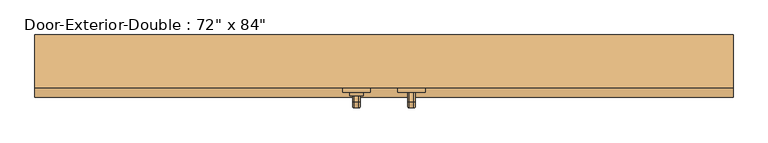
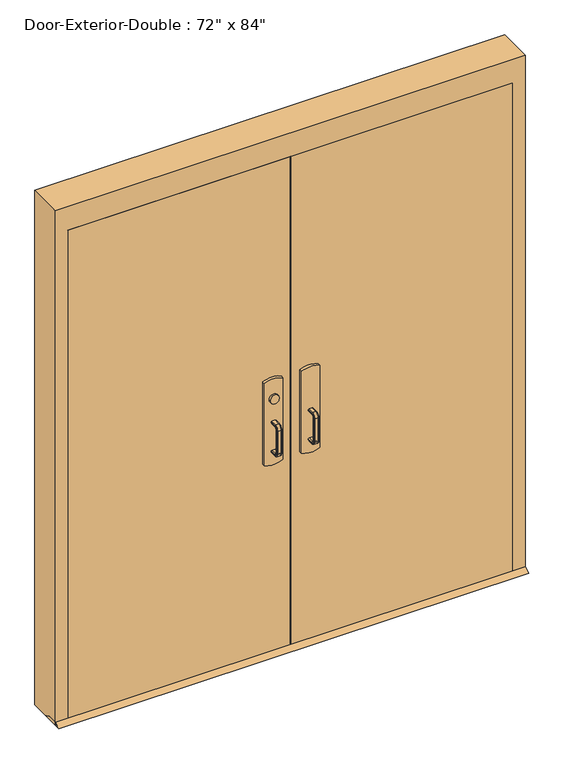
"""IFC4 building model written with IfcOpenShell, lengths in millimetres: door geometry."""

from ifc_helpers import new_model, si_unit, point, frame, frame_2d, origin, place, context, project, spatial, polyline, circle_curve, ellipse_curve, trimmed, segment, composite_curve, outline, extrude, faceted_brep, source, transform, mapped, element, save
from ifc_brep_helpers import plane_surface, cylinder_surface, revolved_surface, advanced_brep


def door_b0164ecf(model_context):
    return source(origin(), model_context, "Body", "SolidModel", [
        extrude(outline(polyline([(-575.7333333, 25.4), (-76.2, 25.4), (-76.2, 19.05), (-575.7333333, 19.05), (-575.7333333, 25.4)])), frame((0.0, 0.0, 990.6), z_axis=(0.0, 0.0, 1.0), x_axis=(1.0, 0.0, 0.0)), (0.0, 0.0, 1.0), 50.8),
        advanced_brep(
        [(-12.7, 19.05, 1041.4), (-12.7, 19.05, 990.6), (-76.2, 19.05, 990.6), (-825.5, 19.05, 990.6), (-825.5, 19.05, 1041.4), (-76.2, 19.05, 1041.4), (-825.5, -12.7, 1041.4), (-825.5, -12.7, 990.6), (-76.2, -12.7, 990.6), (-76.2, -12.7, 927.1), (-57.15, -12.7, 908.05), (-31.75, -12.7, 908.05), (-12.7, -12.7, 927.1), (-12.7, -12.7, 1104.9), (-31.75, -12.7, 1123.95), (-57.15, -12.7, 1123.95), (-76.2, -12.7, 1104.9), (-76.2, -12.7, 1041.4), (-76.2, 15.8747533, 1041.4), (-12.7, 15.8747533, 1041.4), (-12.7, 10.8645731, 1104.9), (-12.7, 10.8645731, 927.1), (-12.7, 15.8747533, 990.6), (-76.2, 15.8747533, 990.6), (-76.2, 10.8645731, 1104.9), (-76.2, 10.8645731, 927.1), (-31.75, 9.361519, 1123.95), (-57.15, 9.361519, 1123.95), (-57.15, 9.361519, 908.05), (-31.75, 9.361519, 908.05)],
        [
            (0, 1),
            (1, 2),
            (2, 3),
            (3, 4),
            (4, 5),
            (5, 0),
            (6, 7),
            (7, 8),
            (8, 9),
            (9, 10, circle_curve(frame((-57.15, -12.7, 927.1), z_axis=(0.0, -1.0, 0.0), x_axis=(-1.0, 0.0, 0.0)), 19.05)),
            (10, 11),
            (11, 12, circle_curve(frame((-31.75, -12.7, 927.1), z_axis=(0.0, -1.0, 0.0), x_axis=(-1.0, 0.0, 0.0)), 19.05)),
            (12, 13),
            (13, 14, circle_curve(frame((-31.75, -12.7, 1104.9), z_axis=(0.0, -1.0, 0.0), x_axis=(-1.0, 0.0, 0.0)), 19.05)),
            (14, 15),
            (15, 16, circle_curve(frame((-57.15, -12.7, 1104.9), z_axis=(0.0, -1.0, 0.0), x_axis=(-1.0, 0.0, 0.0)), 19.05)),
            (16, 17),
            (17, 6),
            (4, 6),
            (17, 18),
            (18, 19),
            (19, 0),
            (19, 20),
            (20, 13),
            (12, 21),
            (21, 22),
            (22, 1),
            (7, 3),
            (22, 23),
            (23, 8),
            (16, 24),
            (24, 18),
            (23, 25),
            (25, 9),
            (14, 26),
            (26, 27),
            (27, 15),
            (10, 28),
            (28, 29),
            (29, 11),
            (25, 28, ellipse_curve(frame((-57.15, 10.8645731, 927.1), z_axis=(0.0, -0.9969018152893365, 0.07865602756830282), x_axis=(0.0, 0.07865602756830208, 0.9969018152893365)), 19.1092038, 19.05)),
            (27, 24, ellipse_curve(frame((-57.15, 10.8645731, 1104.9), z_axis=(0.0, -0.9969018152893376, -0.07865602756828934), x_axis=(0.0, 0.078656027568288, -0.9969018152893377)), 19.1092038, 19.05)),
            (20, 26, ellipse_curve(frame((-31.75, 10.8645731, 1104.9), z_axis=(0.0, -0.9969018152893376, -0.07865602756828934), x_axis=(0.0, 0.078656027568288, -0.9969018152893377)), 19.1092038, 19.05)),
            (29, 21, ellipse_curve(frame((-31.75, 10.8645731, 927.1), z_axis=(0.0, -0.9969018152893365, 0.07865602756830282), x_axis=(0.0, 0.07865602756830208, 0.9969018152893365)), 19.1092038, 19.05)),
        ],
        [
            plane_surface(frame((-12.7, 19.05, 1041.4), z_axis=(0.0, 1.0, 0.0), x_axis=(1.0, 0.0, 0.0))),
            plane_surface(frame((-12.7, -12.7, 1041.4), z_axis=(0.0, -1.0, 0.0), x_axis=(-1.0, 0.0, 0.0))),
            plane_surface(frame((-825.5, 19.05, 1041.4), z_axis=(0.0, 0.0, 1.0), x_axis=(0.0, -1.0, 0.0))),
            plane_surface(frame((-12.7, 19.05, 1041.4), z_axis=(1.0, 0.0, 0.0), x_axis=(0.0, -1.0, 0.0))),
            plane_surface(frame((-12.7, 19.05, 990.6), z_axis=(0.0, 0.0, -1.0), x_axis=(0.0, -1.0, 0.0))),
            plane_surface(frame((-825.5, 19.05, 990.6), z_axis=(-1.0, 0.0, 0.0), x_axis=(0.0, -1.0, 0.0))),
            plane_surface(frame((-76.2, 15.8747533, 927.1), z_axis=(-1.0, 0.0, 0.0), x_axis=(0.0, -1.0, 0.0))),
            plane_surface(frame((-57.15, 15.8747533, 1123.95), z_axis=(0.0, 0.0, 1.0), x_axis=(0.0, -1.0, 0.0))),
            plane_surface(frame((-31.75, 15.8747533, 908.05), z_axis=(0.0, 0.0, -1.0), x_axis=(0.0, -1.0, 0.0))),
            cylinder_surface(frame((-57.15, -12.7, 927.1), z_axis=(0.0, 1.0, 0.0), x_axis=(-1.0, 0.0, 0.0)), 19.05),
            cylinder_surface(frame((-57.15, -12.7, 1104.9), z_axis=(0.0, 1.0, 0.0), x_axis=(-1.0, 0.0, 0.0)), 19.05),
            cylinder_surface(frame((-31.75, -12.7, 1104.9), z_axis=(0.0, 1.0, 0.0), x_axis=(-1.0, 0.0, 0.0)), 19.05),
            cylinder_surface(frame((-31.75, -12.7, 927.1), z_axis=(0.0, 1.0, 0.0), x_axis=(-1.0, 0.0, 0.0)), 19.05),
            plane_surface(frame((-76.2, 15.8747533, 1041.4), z_axis=(0.0, 0.9969018152893376, 0.07865602756828934), x_axis=(1.0, 0.0, 0.0))),
            plane_surface(frame((-76.2, 9.361519, 908.05), z_axis=(0.0, 0.9969018152893365, -0.07865602756830282), x_axis=(1.0, 0.0, 0.0))),
        ],
        [
            (0, [[1, 2, 3, 4, 5, 6]]),
            (1, [[7, 8, 9, 10, 11, 12, 13, 14, 15, 16, 17, 18]]),
            (2, [[19, -18, 20, 21, 22, -6, -5]]),
            (3, [[-1, -22, 23, 24, -13, 25, 26, 27]]),
            (4, [[28, -3, -2, -27, 29, 30, -8]]),
            (5, [[-4, -28, -7, -19]]),
            (6, [[-17, 31, 32, -20]]),
            (6, [[-9, -30, 33, 34]]),
            (7, [[-15, 35, 36, 37]]),
            (8, [[-11, 38, 39, 40]]),
            (9, [[-10, -34, 41, -38]]),
            (10, [[-16, -37, 42, -31]]),
            (11, [[-14, -24, 43, -35]]),
            (12, [[-12, -40, 44, -25]]),
            (13, [[-21, -32, -42, -36, -43, -23]]),
            (14, [[-26, -44, -39, -41, -33, -29]]),
        ],
    ),
        extrude(outline(polyline([(-57.15, 12.7), (-12.7, 12.7), (12.7, 0.0), (-82.55, 0.0), (-57.15, 12.7)])), frame((-965.2, 0.0, 0.0), z_axis=(1.0, 0.0, 0.0), x_axis=(0.0, 1.0, 0.0)), (0.0, 0.0, 1.0), 1930.4),
        extrude(outline(polyline([(575.7333333, 25.4), (575.7333333, 19.05), (76.2, 19.05), (76.2, 25.4), (575.7333333, 25.4)])), frame((0.0, 0.0, 990.6), z_axis=(0.0, 0.0, 1.0), x_axis=(1.0, 0.0, 0.0)), (0.0, 0.0, 1.0), 50.8),
        advanced_brep(
        [(12.7, 19.05, 1041.4), (76.2, 19.05, 1041.4), (825.5, 19.05, 1041.4), (825.5, 19.05, 990.6), (76.2, 19.05, 990.6), (12.7, 19.05, 990.6), (825.5, -12.7, 1041.4), (76.2, -12.7, 1041.4), (76.2, -12.7, 1104.9), (57.15, -12.7, 1123.95), (31.75, -12.7, 1123.95), (12.7, -12.7, 1104.9), (12.7, -12.7, 927.1), (31.75, -12.7, 908.05), (57.15, -12.7, 908.05), (76.2, -12.7, 927.1), (76.2, -12.7, 990.6), (825.5, -12.7, 990.6), (12.7, 15.8747533, 1041.4), (76.2, 15.8747533, 1041.4), (12.7, 15.8747533, 990.6), (12.7, 10.8645731, 927.1), (12.7, 10.8645731, 1104.9), (76.2, 15.8747533, 990.6), (76.2, 10.8645731, 1104.9), (76.2, 10.8645731, 927.1), (57.15, 9.361519, 1123.95), (31.75, 9.361519, 1123.95), (31.75, 9.361519, 908.05), (57.15, 9.361519, 908.05)],
        [
            (0, 1),
            (1, 2),
            (2, 3),
            (3, 4),
            (4, 5),
            (5, 0),
            (6, 7),
            (7, 8),
            (8, 9, circle_curve(frame((57.15, -12.7, 1104.9), z_axis=(0.0, -1.0, 0.0), x_axis=(1.0, 0.0, 0.0)), 19.05)),
            (9, 10),
            (10, 11, circle_curve(frame((31.75, -12.7, 1104.9), z_axis=(0.0, -1.0, 0.0), x_axis=(1.0, 0.0, 0.0)), 19.05)),
            (11, 12),
            (12, 13, circle_curve(frame((31.75, -12.7, 927.1), z_axis=(0.0, -1.0, 0.0), x_axis=(1.0, 0.0, 0.0)), 19.05)),
            (13, 14),
            (14, 15, circle_curve(frame((57.15, -12.7, 927.1), z_axis=(0.0, -1.0, 0.0), x_axis=(1.0, 0.0, 0.0)), 19.05)),
            (15, 16),
            (16, 17),
            (17, 6),
            (0, 18),
            (18, 19),
            (19, 7),
            (6, 2),
            (5, 20),
            (20, 21),
            (21, 12),
            (11, 22),
            (22, 18),
            (16, 23),
            (23, 20),
            (3, 17),
            (19, 24),
            (24, 8),
            (15, 25),
            (25, 23),
            (9, 26),
            (26, 27),
            (27, 10),
            (13, 28),
            (28, 29),
            (29, 14),
            (29, 25, ellipse_curve(frame((57.15, 10.8645731, 927.1), z_axis=(0.0, -0.9969018152893365, 0.07865602756830282), x_axis=(0.0, 0.07865602756830208, 0.9969018152893365)), 19.1092038, 19.05)),
            (24, 26, ellipse_curve(frame((57.15, 10.8645731, 1104.9), z_axis=(0.0, -0.9969018152893376, -0.07865602756828934), x_axis=(0.0, 0.078656027568288, -0.9969018152893377)), 19.1092038, 19.05)),
            (27, 22, ellipse_curve(frame((31.75, 10.8645731, 1104.9), z_axis=(0.0, -0.9969018152893376, -0.07865602756828934), x_axis=(0.0, 0.078656027568288, -0.9969018152893377)), 19.1092038, 19.05)),
            (21, 28, ellipse_curve(frame((31.75, 10.8645731, 927.1), z_axis=(0.0, -0.9969018152893365, 0.07865602756830282), x_axis=(0.0, 0.07865602756830208, 0.9969018152893365)), 19.1092038, 19.05)),
        ],
        [
            plane_surface(frame((12.7, 19.05, 1041.4), z_axis=(0.0, 1.0, 0.0), x_axis=(-1.0, 0.0, 0.0))),
            plane_surface(frame((12.7, -12.7, 1041.4), z_axis=(0.0, -1.0, 0.0), x_axis=(1.0, 0.0, 0.0))),
            plane_surface(frame((825.5, 19.05, 1041.4), z_axis=(0.0, 0.0, 1.0), x_axis=(0.0, -1.0, 0.0))),
            plane_surface(frame((12.7, 19.05, 1041.4), z_axis=(-1.0, 0.0, 0.0), x_axis=(0.0, -1.0, 0.0))),
            plane_surface(frame((12.7, 19.05, 990.6), z_axis=(0.0, 0.0, -1.0), x_axis=(0.0, -1.0, 0.0))),
            plane_surface(frame((825.5, 19.05, 990.6), z_axis=(1.0, 0.0, 0.0), x_axis=(0.0, -1.0, 0.0))),
            plane_surface(frame((76.2, 15.8747533, 927.1), z_axis=(1.0, 0.0, 0.0), x_axis=(0.0, -1.0, 0.0))),
            plane_surface(frame((57.15, 15.8747533, 1123.95), z_axis=(0.0, 0.0, 1.0), x_axis=(0.0, -1.0, 0.0))),
            plane_surface(frame((31.75, 15.8747533, 908.05), z_axis=(0.0, 0.0, -1.0), x_axis=(0.0, -1.0, 0.0))),
            cylinder_surface(frame((57.15, -12.7, 927.1), z_axis=(0.0, 1.0, 0.0), x_axis=(1.0, 0.0, 0.0)), 19.05),
            cylinder_surface(frame((57.15, -12.7, 1104.9), z_axis=(0.0, 1.0, 0.0), x_axis=(1.0, 0.0, 0.0)), 19.05),
            cylinder_surface(frame((31.75, -12.7, 1104.9), z_axis=(0.0, 1.0, 0.0), x_axis=(1.0, 0.0, 0.0)), 19.05),
            cylinder_surface(frame((31.75, -12.7, 927.1), z_axis=(0.0, 1.0, 0.0), x_axis=(1.0, 0.0, 0.0)), 19.05),
            plane_surface(frame((76.2, 15.8747533, 1041.4), z_axis=(0.0, 0.9969018152893376, 0.07865602756828934), x_axis=(-1.0, 0.0, 0.0))),
            plane_surface(frame((76.2, 9.361519, 908.05), z_axis=(0.0, 0.9969018152893365, -0.07865602756830282), x_axis=(-1.0, 0.0, 0.0))),
        ],
        [
            (0, [[1, 2, 3, 4, 5, 6]]),
            (1, [[7, 8, 9, 10, 11, 12, 13, 14, 15, 16, 17, 18]]),
            (2, [[-2, -1, 19, 20, 21, -7, 22]]),
            (3, [[23, 24, 25, -12, 26, 27, -19, -6]]),
            (4, [[-17, 28, 29, -23, -5, -4, 30]]),
            (5, [[-22, -18, -30, -3]]),
            (6, [[-21, 31, 32, -8]]),
            (6, [[33, 34, -28, -16]]),
            (7, [[35, 36, 37, -10]]),
            (8, [[38, 39, 40, -14]]),
            (9, [[-40, 41, -33, -15]]),
            (10, [[-32, 42, -35, -9]]),
            (11, [[-37, 43, -26, -11]]),
            (12, [[-25, 44, -38, -13]]),
            (13, [[-27, -43, -36, -42, -31, -20]]),
            (14, [[-29, -34, -41, -39, -44, -24]]),
        ],
    ),
        advanced_brep(
        [(66.2, -69.85, 1017.190625), (69.771875, -69.85, 1020.7625), (82.628125, -69.85, 1020.7625), (86.2, -69.85, 1017.190625), (86.2, -69.85, 1014.8090406), (82.6284594, -69.85, 1011.2375), (69.771875, -69.85, 1011.2375), (66.2, -69.85, 1014.809375), (66.2, -69.85, 887.809375), (66.2, -69.85, 890.190625), (69.771875, -69.85, 893.7625), (82.6284594, -69.85, 893.7625), (86.2, -69.85, 890.1909594), (86.2, -69.85, 887.809375), (82.628125, -69.85, 884.2375), (69.771875, -69.85, 884.2375), (66.2, -95.25, 1014.809375), (66.2, -106.759375, 1003.3), (66.2, -106.759375, 901.7), (66.2, -95.25, 890.190625), (66.2, -95.25, 887.809375), (66.2, -109.140625, 901.7), (66.2, -109.140625, 1003.3), (66.2, -95.25, 1017.190625), (69.771875, -95.25, 1011.2375), (82.6284594, -95.25, 1011.2375), (86.2, -95.25, 1014.8090406), (86.2, -95.25, 1017.190625), (86.2, -109.140625, 1003.3), (86.2, -109.140625, 901.7), (86.2, -95.25, 887.809375), (86.2, -95.25, 890.1909594), (86.2, -106.7590406, 901.7), (86.2, -106.7590406, 1003.3), (82.628125, -95.25, 1020.7625), (69.771875, -95.25, 1020.7625), (69.771875, -103.1875, 1003.3), (82.6284594, -103.1875, 1003.3), (82.628125, -112.7125, 1003.3), (69.771875, -112.7125, 1003.3), (69.771875, -103.1875, 901.7), (82.6284594, -103.1875, 901.7), (82.628125, -112.7125, 901.7), (69.771875, -112.7125, 901.7), (69.771875, -95.25, 893.7625), (82.6284594, -95.25, 893.7625), (82.628125, -95.25, 884.2375), (69.771875, -95.25, 884.2375)],
        [
            (0, 1, circle_curve(frame((69.771875, -69.85, 1017.190625), z_axis=(0.0, 1.0, 0.0), x_axis=(0.0, 0.0, 1.0)), 3.571875)),
            (1, 2),
            (2, 3, circle_curve(frame((82.628125, -69.85, 1017.190625), z_axis=(0.0, 1.0, 0.0), x_axis=(0.0, 0.0, 1.0)), 3.571875)),
            (3, 4),
            (4, 5, circle_curve(frame((82.6284594, -69.85, 1014.8090406), z_axis=(0.0, 1.0, 0.0), x_axis=(0.0, 0.0, 1.0)), 3.5715406)),
            (5, 6),
            (6, 7, circle_curve(frame((69.771875, -69.85, 1014.809375), z_axis=(0.0, 1.0, 0.0), x_axis=(0.0, 0.0, 1.0)), 3.571875)),
            (7, 0),
            (8, 9),
            (9, 10, circle_curve(frame((69.771875, -69.85, 890.190625), z_axis=(0.0, 1.0, 0.0), x_axis=(0.0, 0.0, -1.0)), 3.571875)),
            (10, 11),
            (11, 12, circle_curve(frame((82.6284594, -69.85, 890.1909594), z_axis=(0.0, 1.0, 0.0), x_axis=(0.0, 0.0, -1.0)), 3.5715406)),
            (12, 13),
            (13, 14, circle_curve(frame((82.628125, -69.85, 887.809375), z_axis=(0.0, 1.0, 0.0), x_axis=(0.0, 0.0, -1.0)), 3.571875)),
            (14, 15),
            (15, 8, circle_curve(frame((69.771875, -69.85, 887.809375), z_axis=(0.0, 1.0, 0.0), x_axis=(0.0, 0.0, -1.0)), 3.571875)),
            (7, 16),
            (16, 17, circle_curve(frame((66.2, -95.25, 1003.3), z_axis=(1.0, 0.0, 0.0), x_axis=(0.0, 0.0, 1.0)), 11.509375)),
            (17, 18),
            (18, 19, circle_curve(frame((66.2, -95.25, 901.7), z_axis=(1.0, 0.0, 0.0), x_axis=(0.0, -1.0, 0.0)), 11.509375)),
            (19, 9),
            (8, 20),
            (20, 21, circle_curve(frame((66.2, -95.25, 901.7), z_axis=(-1.0, 0.0, 0.0), x_axis=(0.0, -1.0, 0.0)), 13.890625)),
            (21, 22),
            (22, 23, circle_curve(frame((66.2, -95.25, 1003.3), z_axis=(-1.0, 0.0, 0.0), x_axis=(0.0, 0.0, 1.0)), 13.890625)),
            (23, 0),
            (6, 24),
            (24, 16, circle_curve(frame((69.771875, -95.25, 1014.809375), z_axis=(0.0, 1.0, 0.0), x_axis=(0.0, 0.0, 1.0)), 3.571875)),
            (5, 25),
            (25, 24),
            (4, 26),
            (26, 25, circle_curve(frame((82.6284594, -95.25, 1014.8090406), z_axis=(0.0, 1.0, 0.0), x_axis=(0.0, 0.0, 1.0)), 3.5715406)),
            (3, 27),
            (27, 28, circle_curve(frame((86.2, -95.25, 1003.3), z_axis=(1.0, 0.0, 0.0), x_axis=(0.0, 0.0, 1.0)), 13.890625)),
            (28, 29),
            (29, 30, circle_curve(frame((86.2, -95.25, 901.7), z_axis=(1.0, 0.0, 0.0), x_axis=(0.0, -1.0, 0.0)), 13.890625)),
            (30, 13),
            (12, 31),
            (31, 32, circle_curve(frame((86.2, -95.25, 901.7), z_axis=(-1.0, 0.0, 0.0), x_axis=(0.0, -1.0, 0.0)), 11.5090406)),
            (32, 33),
            (33, 26, circle_curve(frame((86.2, -95.25, 1003.3), z_axis=(-1.0, 0.0, 0.0), x_axis=(0.0, 0.0, 1.0)), 11.5090406)),
            (2, 34),
            (34, 27, circle_curve(frame((82.628125, -95.25, 1017.190625), z_axis=(0.0, 1.0, 0.0), x_axis=(0.0, 0.0, 1.0)), 3.571875)),
            (1, 35),
            (35, 34),
            (23, 35, circle_curve(frame((69.771875, -95.25, 1017.190625), z_axis=(0.0, 1.0, 0.0), x_axis=(0.0, 0.0, 1.0)), 3.571875)),
            (36, 17, circle_curve(frame((69.771875, -106.759375, 1003.3), z_axis=(0.0, 0.0, 1.0), x_axis=(0.0, -1.0, 0.0)), 3.571875)),
            (24, 36, circle_curve(frame((69.771875, -95.25, 1003.3), z_axis=(1.0, 0.0, 0.0), x_axis=(0.0, 0.0, 1.0)), 7.9375)),
            (37, 36),
            (25, 37, circle_curve(frame((82.6284594, -95.25, 1003.3), z_axis=(1.0, 0.0, 0.0), x_axis=(0.0, 0.0, 1.0)), 7.9375)),
            (33, 37, circle_curve(frame((82.6284594, -106.7590406, 1003.3), z_axis=(0.0, 0.0, 1.0), x_axis=(0.0, -1.0, 0.0)), 3.5715406)),
            (38, 28, circle_curve(frame((82.628125, -109.140625, 1003.3), z_axis=(0.0, 0.0, 1.0), x_axis=(0.0, -1.0, 0.0)), 3.571875)),
            (34, 38, circle_curve(frame((82.628125, -95.25, 1003.3), z_axis=(1.0, 0.0, 0.0), x_axis=(0.0, 0.0, 1.0)), 17.4625)),
            (39, 38),
            (35, 39, circle_curve(frame((69.771875, -95.25, 1003.3), z_axis=(1.0, 0.0, 0.0), x_axis=(0.0, 0.0, 1.0)), 17.4625)),
            (22, 39, circle_curve(frame((69.771875, -109.140625, 1003.3), z_axis=(0.0, 0.0, 1.0), x_axis=(0.0, -1.0, 0.0)), 3.571875)),
            (36, 40),
            (40, 18, circle_curve(frame((69.771875, -106.759375, 901.7), z_axis=(0.0, 0.0, 1.0), x_axis=(0.0, -1.0, 0.0)), 3.571875)),
            (37, 41),
            (41, 40),
            (32, 41, circle_curve(frame((82.6284594, -106.7590406, 901.7), z_axis=(0.0, 0.0, 1.0), x_axis=(0.0, -1.0, 0.0)), 3.5715406)),
            (38, 42),
            (42, 29, circle_curve(frame((82.628125, -109.140625, 901.7), z_axis=(0.0, 0.0, 1.0), x_axis=(0.0, -1.0, 0.0)), 3.571875)),
            (39, 43),
            (43, 42),
            (21, 43, circle_curve(frame((69.771875, -109.140625, 901.7), z_axis=(0.0, 0.0, 1.0), x_axis=(0.0, -1.0, 0.0)), 3.571875)),
            (44, 19, circle_curve(frame((69.771875, -95.25, 890.190625), z_axis=(0.0, -1.0, 0.0), x_axis=(0.0, 0.0, -1.0)), 3.571875)),
            (40, 44, circle_curve(frame((69.771875, -95.25, 901.7), z_axis=(1.0, 0.0, 0.0), x_axis=(0.0, -1.0, 0.0)), 7.9375)),
            (45, 44),
            (41, 45, circle_curve(frame((82.6284594, -95.25, 901.7), z_axis=(1.0, 0.0, 0.0), x_axis=(0.0, -1.0, 0.0)), 7.9375)),
            (31, 45, circle_curve(frame((82.6284594, -95.25, 890.1909594), z_axis=(0.0, -1.0, 0.0), x_axis=(0.0, 0.0, -1.0)), 3.5715406)),
            (46, 30, circle_curve(frame((82.628125, -95.25, 887.809375), z_axis=(0.0, -1.0, 0.0), x_axis=(0.0, 0.0, -1.0)), 3.571875)),
            (42, 46, circle_curve(frame((82.628125, -95.25, 901.7), z_axis=(1.0, 0.0, 0.0), x_axis=(0.0, -1.0, 0.0)), 17.4625)),
            (47, 46),
            (43, 47, circle_curve(frame((69.771875, -95.25, 901.7), z_axis=(1.0, 0.0, 0.0), x_axis=(0.0, -1.0, 0.0)), 17.4625)),
            (20, 47, circle_curve(frame((69.771875, -95.25, 887.809375), z_axis=(0.0, -1.0, 0.0), x_axis=(0.0, 0.0, -1.0)), 3.571875)),
            (44, 10),
            (45, 11),
            (46, 14),
            (47, 15),
        ],
        [
            plane_surface(frame((76.2, -69.85, 1016.0), z_axis=(0.0, 1.0, 0.0), x_axis=(1.0, 0.0, 0.0))),
            plane_surface(frame((76.2, -69.85, 889.0), z_axis=(0.0, 1.0, 0.0), x_axis=(1.0, 0.0, 0.0))),
            plane_surface(frame((66.2, -69.85, 1017.190625), z_axis=(-1.0, 0.0, 0.0), x_axis=(0.0, -1.0, 0.0))),
            cylinder_surface(frame((69.771875, -69.85, 1014.809375), z_axis=(0.0, 1.0, 0.0), x_axis=(0.0, 0.0, 1.0)), 3.571875),
            plane_surface(frame((69.771875, -69.85, 1011.2375), z_axis=(0.0, 0.0, -1.0), x_axis=(0.0, -1.0, 0.0))),
            cylinder_surface(frame((82.6284594, -69.85, 1014.8090406), z_axis=(0.0, 1.0, 0.0), x_axis=(0.0, 0.0, 1.0)), 3.5715406),
            plane_surface(frame((86.2, -69.85, 1014.8090406), z_axis=(1.0, 0.0, 0.0), x_axis=(0.0, -1.0, 0.0))),
            cylinder_surface(frame((82.628125, -69.85, 1017.190625), z_axis=(0.0, 1.0, 0.0), x_axis=(0.0, 0.0, 1.0)), 3.571875),
            plane_surface(frame((82.628125, -69.85, 1020.7625), z_axis=(0.0, 0.0, 1.0), x_axis=(0.0, -1.0, 0.0))),
            cylinder_surface(frame((69.771875, -69.85, 1017.190625), z_axis=(0.0, 1.0, 0.0), x_axis=(0.0, 0.0, 1.0)), 3.571875),
            revolved_surface(trimmed(ellipse_curve(frame((69.771875, -95.25, 1014.809375), z_axis=(0.0, -1.0, 0.0), x_axis=(0.0, 0.0, 1.0)), 3.571875, 3.571875), [point((66.2, -95.25, 1014.809375))], [point((69.771875, -95.25, 1011.2375))], True, "CARTESIAN"), (76.2, -95.25, 1003.3), (-1.0, 0.0, 0.0)),
            revolved_surface(polyline([(69.771875, -95.25, 1011.2375), (82.6284594, -95.25, 1011.2375)]), (76.2, -95.25, 1003.3), (-1.0, 0.0, 0.0)),
            revolved_surface(trimmed(ellipse_curve(frame((82.6284594, -95.25, 1014.8090406), z_axis=(0.0, -1.0, 0.0), x_axis=(0.0, 0.0, 1.0)), 3.5715406, 3.5715406), [point((82.6284594, -95.25, 1011.2375))], [point((86.2, -95.25, 1014.8090406))], True, "CARTESIAN"), (76.2, -95.25, 1003.3), (-1.0, 0.0, 0.0)),
            revolved_surface(trimmed(ellipse_curve(frame((82.628125, -95.25, 1017.190625), z_axis=(0.0, -1.0, 0.0), x_axis=(0.0, 0.0, 1.0)), 3.571875, 3.571875), [point((86.2, -95.25, 1017.190625))], [point((82.628125, -95.25, 1020.7625))], True, "CARTESIAN"), (76.2, -95.25, 1003.3), (-1.0, 0.0, 0.0)),
            cylinder_surface(frame((76.2, -95.25, 1003.3), z_axis=(-1.0, 0.0, 0.0), x_axis=(0.0, 0.0, 1.0)), 17.4625),
            revolved_surface(trimmed(ellipse_curve(frame((69.771875, -95.25, 1017.190625), z_axis=(0.0, -1.0, 0.0), x_axis=(0.0, 0.0, 1.0)), 3.571875, 3.571875), [point((69.771875, -95.25, 1020.7625))], [point((66.2, -95.25, 1017.190625))], True, "CARTESIAN"), (76.2, -95.25, 1003.3), (-1.0, 0.0, 0.0)),
            cylinder_surface(frame((69.771875, -106.759375, 1003.3), z_axis=(0.0, 0.0, 1.0), x_axis=(0.0, -1.0, 0.0)), 3.571875),
            plane_surface(frame((69.771875, -103.1875, 1003.3), z_axis=(0.0, 1.0, 0.0), x_axis=(0.0, 0.0, -1.0))),
            cylinder_surface(frame((82.6284594, -106.7590406, 1003.3), z_axis=(0.0, 0.0, 1.0), x_axis=(0.0, -1.0, 0.0)), 3.5715406),
            cylinder_surface(frame((82.628125, -109.140625, 1003.3), z_axis=(0.0, 0.0, 1.0), x_axis=(0.0, -1.0, 0.0)), 3.571875),
            plane_surface(frame((82.628125, -112.7125, 1003.3), z_axis=(0.0, -1.0, 0.0), x_axis=(0.0, 0.0, -1.0))),
            cylinder_surface(frame((69.771875, -109.140625, 1003.3), z_axis=(0.0, 0.0, 1.0), x_axis=(0.0, -1.0, 0.0)), 3.571875),
            revolved_surface(trimmed(ellipse_curve(frame((69.771875, -106.759375, 901.7), z_axis=(0.0, 0.0, -1.0), x_axis=(0.0, -1.0, 0.0)), 3.571875, 3.571875), [point((66.2, -106.759375, 901.7))], [point((69.771875, -103.1875, 901.7))], True, "CARTESIAN"), (76.2, -95.25, 901.7), (-1.0, 0.0, 0.0)),
            revolved_surface(polyline([(69.771875, -103.1875, 901.7), (82.6284594, -103.1875, 901.7)]), (76.2, -95.25, 901.7), (-1.0, 0.0, 0.0)),
            revolved_surface(trimmed(ellipse_curve(frame((82.6284594, -106.7590406, 901.7), z_axis=(0.0, 0.0, -1.0), x_axis=(0.0, -1.0, 0.0)), 3.5715406, 3.5715406), [point((82.6284594, -103.1875, 901.7))], [point((86.2, -106.7590406, 901.7))], True, "CARTESIAN"), (76.2, -95.25, 901.7), (-1.0, 0.0, 0.0)),
            revolved_surface(trimmed(ellipse_curve(frame((82.628125, -109.140625, 901.7), z_axis=(0.0, 0.0, -1.0), x_axis=(0.0, -1.0, 0.0)), 3.571875, 3.571875), [point((86.2, -109.140625, 901.7))], [point((82.628125, -112.7125, 901.7))], True, "CARTESIAN"), (76.2, -95.25, 901.7), (-1.0, 0.0, 0.0)),
            cylinder_surface(frame((76.2, -95.25, 901.7), z_axis=(-1.0, 0.0, 0.0), x_axis=(0.0, -1.0, 0.0)), 17.4625),
            revolved_surface(trimmed(ellipse_curve(frame((69.771875, -109.140625, 901.7), z_axis=(0.0, 0.0, -1.0), x_axis=(0.0, -1.0, 0.0)), 3.571875, 3.571875), [point((69.771875, -112.7125, 901.7))], [point((66.2, -109.140625, 901.7))], True, "CARTESIAN"), (76.2, -95.25, 901.7), (-1.0, 0.0, 0.0)),
            cylinder_surface(frame((69.771875, -95.25, 890.190625), z_axis=(0.0, -1.0, 0.0), x_axis=(0.0, 0.0, -1.0)), 3.571875),
            plane_surface(frame((69.771875, -95.25, 893.7625), z_axis=(0.0, 0.0, 1.0), x_axis=(0.0, 1.0, 0.0))),
            cylinder_surface(frame((82.6284594, -95.25, 890.1909594), z_axis=(0.0, -1.0, 0.0), x_axis=(0.0, 0.0, -1.0)), 3.5715406),
            cylinder_surface(frame((82.628125, -95.25, 887.809375), z_axis=(0.0, -1.0, 0.0), x_axis=(0.0, 0.0, -1.0)), 3.571875),
            plane_surface(frame((82.628125, -95.25, 884.2375), z_axis=(0.0, 0.0, -1.0), x_axis=(0.0, 1.0, 0.0))),
            cylinder_surface(frame((69.771875, -95.25, 887.809375), z_axis=(0.0, -1.0, 0.0), x_axis=(0.0, 0.0, -1.0)), 3.571875),
        ],
        [
            (0, [[1, 2, 3, 4, 5, 6, 7, 8]]),
            (1, [[9, 10, 11, 12, 13, 14, 15, 16]]),
            (2, [[17, 18, 19, 20, 21, -9, 22, 23, 24, 25, 26, -8]]),
            (3, [[27, 28, -17, -7]]),
            (4, [[29, 30, -27, -6]]),
            (5, [[31, 32, -29, -5]]),
            (6, [[33, 34, 35, 36, 37, -13, 38, 39, 40, 41, -31, -4]]),
            (7, [[42, 43, -33, -3]]),
            (8, [[44, 45, -42, -2]]),
            (9, [[-26, 46, -44, -1]]),
            (10, [[47, -18, -28, 48]]),
            (11, [[49, -48, -30, 50]]),
            (12, [[51, -50, -32, -41]]),
            (13, [[52, -34, -43, 53]]),
            (14, [[54, -53, -45, 55]]),
            (15, [[56, -55, -46, -25]]),
            (16, [[57, 58, -19, -47]]),
            (17, [[59, 60, -57, -49]]),
            (18, [[-40, 61, -59, -51]]),
            (19, [[62, 63, -35, -52]]),
            (20, [[64, 65, -62, -54]]),
            (21, [[-24, 66, -64, -56]]),
            (22, [[67, -20, -58, 68]]),
            (23, [[69, -68, -60, 70]]),
            (24, [[71, -70, -61, -39]]),
            (25, [[72, -36, -63, 73]]),
            (26, [[74, -73, -65, 75]]),
            (27, [[76, -75, -66, -23]]),
            (28, [[77, -10, -21, -67]]),
            (29, [[78, -11, -77, -69]]),
            (30, [[-38, -12, -78, -71]]),
            (31, [[79, -14, -37, -72]]),
            (32, [[80, -15, -79, -74]]),
            (33, [[-22, -16, -80, -76]]),
        ],
    ),
        extrude(outline(composite_curve([segment(trimmed(circle_curve(frame_2d((1113.0338574, 76.2)), 89.3016225), [point((1193.8, 114.3))], [point((1193.8, 38.1))], False, "CARTESIAN"), True, "CONTINUOUS"), segment(polyline([(1193.8, 38.1), (838.2, 38.1)]), True, "CONTINUOUS"), segment(trimmed(circle_curve(frame_2d((918.9661426, 76.2)), 89.3016225), [point((838.2, 38.1))], [point((838.2, 114.3))], False, "CARTESIAN"), True, "CONTINUOUS"), segment(polyline([(838.2, 114.3), (1193.8, 114.3)]), True, "CONTINUOUS")], self_intersect=False)), frame((0.0, -69.85, 0.0), z_axis=(0.0, 1.0, 0.0), x_axis=(0.0, 0.0, 1.0)), (0.0, 0.0, 1.0), 12.7),
        advanced_brep(
        [(-86.2, -69.85, 1017.190625), (-82.628125, -69.85, 1020.7625), (-69.771875, -69.85, 1020.7625), (-66.2, -69.85, 1017.190625), (-66.2, -69.85, 1014.8090406), (-69.7715406, -69.85, 1011.2375), (-82.628125, -69.85, 1011.2375), (-86.2, -69.85, 1014.809375), (-86.2, -69.85, 887.809375), (-86.2, -69.85, 890.190625), (-82.628125, -69.85, 893.7625), (-69.7715406, -69.85, 893.7625), (-66.2, -69.85, 890.1909594), (-66.2, -69.85, 887.809375), (-69.771875, -69.85, 884.2375), (-82.628125, -69.85, 884.2375), (-86.2, -95.25, 1014.809375), (-86.2, -106.759375, 1003.3), (-86.2, -106.759375, 901.7), (-86.2, -95.25, 890.190625), (-86.2, -95.25, 887.809375), (-86.2, -109.140625, 901.7), (-86.2, -109.140625, 1003.3), (-86.2, -95.25, 1017.190625), (-82.628125, -95.25, 1011.2375), (-69.7715406, -95.25, 1011.2375), (-66.2, -95.25, 1014.8090406), (-66.2, -95.25, 1017.190625), (-66.2, -109.140625, 1003.3), (-66.2, -109.140625, 901.7), (-66.2, -95.25, 887.809375), (-66.2, -95.25, 890.1909594), (-66.2, -106.7590406, 901.7), (-66.2, -106.7590406, 1003.3), (-69.771875, -95.25, 1020.7625), (-82.628125, -95.25, 1020.7625), (-82.628125, -103.1875, 1003.3), (-69.7715406, -103.1875, 1003.3), (-69.771875, -112.7125, 1003.3), (-82.628125, -112.7125, 1003.3), (-82.628125, -103.1875, 901.7), (-69.7715406, -103.1875, 901.7), (-69.771875, -112.7125, 901.7), (-82.628125, -112.7125, 901.7), (-82.628125, -95.25, 893.7625), (-69.7715406, -95.25, 893.7625), (-69.771875, -95.25, 884.2375), (-82.628125, -95.25, 884.2375)],
        [
            (0, 1, circle_curve(frame((-82.628125, -69.85, 1017.190625), z_axis=(0.0, 1.0, 0.0), x_axis=(0.0, 0.0, 1.0)), 3.571875)),
            (1, 2),
            (2, 3, circle_curve(frame((-69.771875, -69.85, 1017.190625), z_axis=(0.0, 1.0, 0.0), x_axis=(0.0, 0.0, 1.0)), 3.571875)),
            (3, 4),
            (4, 5, circle_curve(frame((-69.7715406, -69.85, 1014.8090406), z_axis=(0.0, 1.0, 0.0), x_axis=(0.0, 0.0, 1.0)), 3.5715406)),
            (5, 6),
            (6, 7, circle_curve(frame((-82.628125, -69.85, 1014.809375), z_axis=(0.0, 1.0, 0.0), x_axis=(0.0, 0.0, 1.0)), 3.571875)),
            (7, 0),
            (8, 9),
            (9, 10, circle_curve(frame((-82.628125, -69.85, 890.190625), z_axis=(0.0, 1.0, 0.0), x_axis=(0.0, 0.0, -1.0)), 3.571875)),
            (10, 11),
            (11, 12, circle_curve(frame((-69.7715406, -69.85, 890.1909594), z_axis=(0.0, 1.0, 0.0), x_axis=(0.0, 0.0, -1.0)), 3.5715406)),
            (12, 13),
            (13, 14, circle_curve(frame((-69.771875, -69.85, 887.809375), z_axis=(0.0, 1.0, 0.0), x_axis=(0.0, 0.0, -1.0)), 3.571875)),
            (14, 15),
            (15, 8, circle_curve(frame((-82.628125, -69.85, 887.809375), z_axis=(0.0, 1.0, 0.0), x_axis=(0.0, 0.0, -1.0)), 3.571875)),
            (7, 16),
            (16, 17, circle_curve(frame((-86.2, -95.25, 1003.3), z_axis=(1.0, 0.0, 0.0), x_axis=(0.0, 0.0, 1.0)), 11.509375)),
            (17, 18),
            (18, 19, circle_curve(frame((-86.2, -95.25, 901.7), z_axis=(1.0, 0.0, 0.0), x_axis=(0.0, -1.0, 0.0)), 11.509375)),
            (19, 9),
            (8, 20),
            (20, 21, circle_curve(frame((-86.2, -95.25, 901.7), z_axis=(-1.0, 0.0, 0.0), x_axis=(0.0, -1.0, 0.0)), 13.890625)),
            (21, 22),
            (22, 23, circle_curve(frame((-86.2, -95.25, 1003.3), z_axis=(-1.0, 0.0, 0.0), x_axis=(0.0, 0.0, 1.0)), 13.890625)),
            (23, 0),
            (6, 24),
            (24, 16, circle_curve(frame((-82.628125, -95.25, 1014.809375), z_axis=(0.0, 1.0, 0.0), x_axis=(0.0, 0.0, 1.0)), 3.571875)),
            (5, 25),
            (25, 24),
            (4, 26),
            (26, 25, circle_curve(frame((-69.7715406, -95.25, 1014.8090406), z_axis=(0.0, 1.0, 0.0), x_axis=(0.0, 0.0, 1.0)), 3.5715406)),
            (3, 27),
            (27, 28, circle_curve(frame((-66.2, -95.25, 1003.3), z_axis=(1.0, 0.0, 0.0), x_axis=(0.0, 0.0, 1.0)), 13.890625)),
            (28, 29),
            (29, 30, circle_curve(frame((-66.2, -95.25, 901.7), z_axis=(1.0, 0.0, 0.0), x_axis=(0.0, -1.0, 0.0)), 13.890625)),
            (30, 13),
            (12, 31),
            (31, 32, circle_curve(frame((-66.2, -95.25, 901.7), z_axis=(-1.0, 0.0, 0.0), x_axis=(0.0, -1.0, 0.0)), 11.5090406)),
            (32, 33),
            (33, 26, circle_curve(frame((-66.2, -95.25, 1003.3), z_axis=(-1.0, 0.0, 0.0), x_axis=(0.0, 0.0, 1.0)), 11.5090406)),
            (2, 34),
            (34, 27, circle_curve(frame((-69.771875, -95.25, 1017.190625), z_axis=(0.0, 1.0, 0.0), x_axis=(0.0, 0.0, 1.0)), 3.571875)),
            (1, 35),
            (35, 34),
            (23, 35, circle_curve(frame((-82.628125, -95.25, 1017.190625), z_axis=(0.0, 1.0, 0.0), x_axis=(0.0, 0.0, 1.0)), 3.571875)),
            (36, 17, circle_curve(frame((-82.628125, -106.759375, 1003.3), z_axis=(0.0, 0.0, 1.0), x_axis=(0.0, -1.0, 0.0)), 3.571875)),
            (24, 36, circle_curve(frame((-82.628125, -95.25, 1003.3), z_axis=(1.0, 0.0, 0.0), x_axis=(0.0, 0.0, 1.0)), 7.9375)),
            (37, 36),
            (25, 37, circle_curve(frame((-69.7715406, -95.25, 1003.3), z_axis=(1.0, 0.0, 0.0), x_axis=(0.0, 0.0, 1.0)), 7.9375)),
            (33, 37, circle_curve(frame((-69.7715406, -106.7590406, 1003.3), z_axis=(0.0, 0.0, 1.0), x_axis=(0.0, -1.0, 0.0)), 3.5715406)),
            (38, 28, circle_curve(frame((-69.771875, -109.140625, 1003.3), z_axis=(0.0, 0.0, 1.0), x_axis=(0.0, -1.0, 0.0)), 3.571875)),
            (34, 38, circle_curve(frame((-69.771875, -95.25, 1003.3), z_axis=(1.0, 0.0, 0.0), x_axis=(0.0, 0.0, 1.0)), 17.4625)),
            (39, 38),
            (35, 39, circle_curve(frame((-82.628125, -95.25, 1003.3), z_axis=(1.0, 0.0, 0.0), x_axis=(0.0, 0.0, 1.0)), 17.4625)),
            (22, 39, circle_curve(frame((-82.628125, -109.140625, 1003.3), z_axis=(0.0, 0.0, 1.0), x_axis=(0.0, -1.0, 0.0)), 3.571875)),
            (36, 40),
            (40, 18, circle_curve(frame((-82.628125, -106.759375, 901.7), z_axis=(0.0, 0.0, 1.0), x_axis=(0.0, -1.0, 0.0)), 3.571875)),
            (37, 41),
            (41, 40),
            (32, 41, circle_curve(frame((-69.7715406, -106.7590406, 901.7), z_axis=(0.0, 0.0, 1.0), x_axis=(0.0, -1.0, 0.0)), 3.5715406)),
            (38, 42),
            (42, 29, circle_curve(frame((-69.771875, -109.140625, 901.7), z_axis=(0.0, 0.0, 1.0), x_axis=(0.0, -1.0, 0.0)), 3.571875)),
            (39, 43),
            (43, 42),
            (21, 43, circle_curve(frame((-82.628125, -109.140625, 901.7), z_axis=(0.0, 0.0, 1.0), x_axis=(0.0, -1.0, 0.0)), 3.571875)),
            (44, 19, circle_curve(frame((-82.628125, -95.25, 890.190625), z_axis=(0.0, -1.0, 0.0), x_axis=(0.0, 0.0, -1.0)), 3.571875)),
            (40, 44, circle_curve(frame((-82.628125, -95.25, 901.7), z_axis=(1.0, 0.0, 0.0), x_axis=(0.0, -1.0, 0.0)), 7.9375)),
            (45, 44),
            (41, 45, circle_curve(frame((-69.7715406, -95.25, 901.7), z_axis=(1.0, 0.0, 0.0), x_axis=(0.0, -1.0, 0.0)), 7.9375)),
            (31, 45, circle_curve(frame((-69.7715406, -95.25, 890.1909594), z_axis=(0.0, -1.0, 0.0), x_axis=(0.0, 0.0, -1.0)), 3.5715406)),
            (46, 30, circle_curve(frame((-69.771875, -95.25, 887.809375), z_axis=(0.0, -1.0, 0.0), x_axis=(0.0, 0.0, -1.0)), 3.571875)),
            (42, 46, circle_curve(frame((-69.771875, -95.25, 901.7), z_axis=(1.0, 0.0, 0.0), x_axis=(0.0, -1.0, 0.0)), 17.4625)),
            (47, 46),
            (43, 47, circle_curve(frame((-82.628125, -95.25, 901.7), z_axis=(1.0, 0.0, 0.0), x_axis=(0.0, -1.0, 0.0)), 17.4625)),
            (20, 47, circle_curve(frame((-82.628125, -95.25, 887.809375), z_axis=(0.0, -1.0, 0.0), x_axis=(0.0, 0.0, -1.0)), 3.571875)),
            (44, 10),
            (45, 11),
            (46, 14),
            (47, 15),
        ],
        [
            plane_surface(frame((-76.2, -69.85, 1016.0), z_axis=(0.0, 1.0, 0.0), x_axis=(1.0, 0.0, 0.0))),
            plane_surface(frame((-76.2, -69.85, 889.0), z_axis=(0.0, 1.0, 0.0), x_axis=(1.0, 0.0, 0.0))),
            plane_surface(frame((-86.2, -69.85, 1017.190625), z_axis=(-1.0, 0.0, 0.0), x_axis=(0.0, -1.0, 0.0))),
            cylinder_surface(frame((-82.628125, -69.85, 1014.809375), z_axis=(0.0, 1.0, 0.0), x_axis=(0.0, 0.0, 1.0)), 3.571875),
            plane_surface(frame((-82.628125, -69.85, 1011.2375), z_axis=(0.0, 0.0, -1.0), x_axis=(0.0, -1.0, 0.0))),
            cylinder_surface(frame((-69.7715406, -69.85, 1014.8090406), z_axis=(0.0, 1.0, 0.0), x_axis=(0.0, 0.0, 1.0)), 3.5715406),
            plane_surface(frame((-66.2, -69.85, 1014.8090406), z_axis=(1.0, 0.0, 0.0), x_axis=(0.0, -1.0, 0.0))),
            cylinder_surface(frame((-69.771875, -69.85, 1017.190625), z_axis=(0.0, 1.0, 0.0), x_axis=(0.0, 0.0, 1.0)), 3.571875),
            plane_surface(frame((-69.771875, -69.85, 1020.7625), z_axis=(0.0, 0.0, 1.0), x_axis=(0.0, -1.0, 0.0))),
            cylinder_surface(frame((-82.628125, -69.85, 1017.190625), z_axis=(0.0, 1.0, 0.0), x_axis=(0.0, 0.0, 1.0)), 3.571875),
            revolved_surface(trimmed(ellipse_curve(frame((-82.628125, -95.25, 1014.809375), z_axis=(0.0, -1.0, 0.0), x_axis=(0.0, 0.0, 1.0)), 3.571875, 3.571875), [point((-86.2, -95.25, 1014.809375))], [point((-82.628125, -95.25, 1011.2375))], True, "CARTESIAN"), (-76.2, -95.25, 1003.3), (-1.0, 0.0, 0.0)),
            revolved_surface(polyline([(-82.628125, -95.25, 1011.2375), (-69.7715406, -95.25, 1011.2375)]), (-76.2, -95.25, 1003.3), (-1.0, 0.0, 0.0)),
            revolved_surface(trimmed(ellipse_curve(frame((-69.7715406, -95.25, 1014.8090406), z_axis=(0.0, -1.0, 0.0), x_axis=(0.0, 0.0, 1.0)), 3.5715406, 3.5715406), [point((-69.7715406, -95.25, 1011.2375))], [point((-66.2, -95.25, 1014.8090406))], True, "CARTESIAN"), (-76.2, -95.25, 1003.3), (-1.0, 0.0, 0.0)),
            revolved_surface(trimmed(ellipse_curve(frame((-69.771875, -95.25, 1017.190625), z_axis=(0.0, -1.0, 0.0), x_axis=(0.0, 0.0, 1.0)), 3.571875, 3.571875), [point((-66.2, -95.25, 1017.190625))], [point((-69.771875, -95.25, 1020.7625))], True, "CARTESIAN"), (-76.2, -95.25, 1003.3), (-1.0, 0.0, 0.0)),
            cylinder_surface(frame((-76.2, -95.25, 1003.3), z_axis=(-1.0, 0.0, 0.0), x_axis=(0.0, 0.0, 1.0)), 17.4625),
            revolved_surface(trimmed(ellipse_curve(frame((-82.628125, -95.25, 1017.190625), z_axis=(0.0, -1.0, 0.0), x_axis=(0.0, 0.0, 1.0)), 3.571875, 3.571875), [point((-82.628125, -95.25, 1020.7625))], [point((-86.2, -95.25, 1017.190625))], True, "CARTESIAN"), (-76.2, -95.25, 1003.3), (-1.0, 0.0, 0.0)),
            cylinder_surface(frame((-82.628125, -106.759375, 1003.3), z_axis=(0.0, 0.0, 1.0), x_axis=(0.0, -1.0, 0.0)), 3.571875),
            plane_surface(frame((-82.628125, -103.1875, 1003.3), z_axis=(0.0, 1.0, 0.0), x_axis=(0.0, 0.0, -1.0))),
            cylinder_surface(frame((-69.7715406, -106.7590406, 1003.3), z_axis=(0.0, 0.0, 1.0), x_axis=(0.0, -1.0, 0.0)), 3.5715406),
            cylinder_surface(frame((-69.771875, -109.140625, 1003.3), z_axis=(0.0, 0.0, 1.0), x_axis=(0.0, -1.0, 0.0)), 3.571875),
            plane_surface(frame((-69.771875, -112.7125, 1003.3), z_axis=(0.0, -1.0, 0.0), x_axis=(0.0, 0.0, -1.0))),
            cylinder_surface(frame((-82.628125, -109.140625, 1003.3), z_axis=(0.0, 0.0, 1.0), x_axis=(0.0, -1.0, 0.0)), 3.571875),
            revolved_surface(trimmed(ellipse_curve(frame((-82.628125, -106.759375, 901.7), z_axis=(0.0, 0.0, -1.0), x_axis=(0.0, -1.0, 0.0)), 3.571875, 3.571875), [point((-86.2, -106.759375, 901.7))], [point((-82.628125, -103.1875, 901.7))], True, "CARTESIAN"), (-76.2, -95.25, 901.7), (-1.0, 0.0, 0.0)),
            revolved_surface(polyline([(-82.628125, -103.1875, 901.7), (-69.7715406, -103.1875, 901.7)]), (-76.2, -95.25, 901.7), (-1.0, 0.0, 0.0)),
            revolved_surface(trimmed(ellipse_curve(frame((-69.7715406, -106.7590406, 901.7), z_axis=(0.0, 0.0, -1.0), x_axis=(0.0, -1.0, 0.0)), 3.5715406, 3.5715406), [point((-69.7715406, -103.1875, 901.7))], [point((-66.2, -106.7590406, 901.7))], True, "CARTESIAN"), (-76.2, -95.25, 901.7), (-1.0, 0.0, 0.0)),
            revolved_surface(trimmed(ellipse_curve(frame((-69.771875, -109.140625, 901.7), z_axis=(0.0, 0.0, -1.0), x_axis=(0.0, -1.0, 0.0)), 3.571875, 3.571875), [point((-66.2, -109.140625, 901.7))], [point((-69.771875, -112.7125, 901.7))], True, "CARTESIAN"), (-76.2, -95.25, 901.7), (-1.0, 0.0, 0.0)),
            cylinder_surface(frame((-76.2, -95.25, 901.7), z_axis=(-1.0, 0.0, 0.0), x_axis=(0.0, -1.0, 0.0)), 17.4625),
            revolved_surface(trimmed(ellipse_curve(frame((-82.628125, -109.140625, 901.7), z_axis=(0.0, 0.0, -1.0), x_axis=(0.0, -1.0, 0.0)), 3.571875, 3.571875), [point((-82.628125, -112.7125, 901.7))], [point((-86.2, -109.140625, 901.7))], True, "CARTESIAN"), (-76.2, -95.25, 901.7), (-1.0, 0.0, 0.0)),
            cylinder_surface(frame((-82.628125, -95.25, 890.190625), z_axis=(0.0, -1.0, 0.0), x_axis=(0.0, 0.0, -1.0)), 3.571875),
            plane_surface(frame((-82.628125, -95.25, 893.7625), z_axis=(0.0, 0.0, 1.0), x_axis=(0.0, 1.0, 0.0))),
            cylinder_surface(frame((-69.7715406, -95.25, 890.1909594), z_axis=(0.0, -1.0, 0.0), x_axis=(0.0, 0.0, -1.0)), 3.5715406),
            cylinder_surface(frame((-69.771875, -95.25, 887.809375), z_axis=(0.0, -1.0, 0.0), x_axis=(0.0, 0.0, -1.0)), 3.571875),
            plane_surface(frame((-69.771875, -95.25, 884.2375), z_axis=(0.0, 0.0, -1.0), x_axis=(0.0, 1.0, 0.0))),
            cylinder_surface(frame((-82.628125, -95.25, 887.809375), z_axis=(0.0, -1.0, 0.0), x_axis=(0.0, 0.0, -1.0)), 3.571875),
        ],
        [
            (0, [[1, 2, 3, 4, 5, 6, 7, 8]]),
            (1, [[9, 10, 11, 12, 13, 14, 15, 16]]),
            (2, [[17, 18, 19, 20, 21, -9, 22, 23, 24, 25, 26, -8]]),
            (3, [[27, 28, -17, -7]]),
            (4, [[29, 30, -27, -6]]),
            (5, [[31, 32, -29, -5]]),
            (6, [[33, 34, 35, 36, 37, -13, 38, 39, 40, 41, -31, -4]]),
            (7, [[42, 43, -33, -3]]),
            (8, [[44, 45, -42, -2]]),
            (9, [[-26, 46, -44, -1]]),
            (10, [[47, -18, -28, 48]]),
            (11, [[49, -48, -30, 50]]),
            (12, [[51, -50, -32, -41]]),
            (13, [[52, -34, -43, 53]]),
            (14, [[54, -53, -45, 55]]),
            (15, [[56, -55, -46, -25]]),
            (16, [[57, 58, -19, -47]]),
            (17, [[59, 60, -57, -49]]),
            (18, [[-40, 61, -59, -51]]),
            (19, [[62, 63, -35, -52]]),
            (20, [[64, 65, -62, -54]]),
            (21, [[-24, 66, -64, -56]]),
            (22, [[67, -20, -58, 68]]),
            (23, [[69, -68, -60, 70]]),
            (24, [[71, -70, -61, -39]]),
            (25, [[72, -36, -63, 73]]),
            (26, [[74, -73, -65, 75]]),
            (27, [[76, -75, -66, -23]]),
            (28, [[77, -10, -21, -67]]),
            (29, [[78, -11, -77, -69]]),
            (30, [[-38, -12, -78, -71]]),
            (31, [[79, -14, -37, -72]]),
            (32, [[80, -15, -79, -74]]),
            (33, [[-22, -16, -80, -76]]),
        ],
    ),
        extrude(outline(composite_curve([segment(trimmed(circle_curve(frame_2d((1117.6, -76.2)), 19.0), [point((1117.6, -95.2))], [point((1117.6, -57.2))], False, "CARTESIAN"), True, "CONTINUOUS"), segment(trimmed(circle_curve(frame_2d((1117.6, -76.2)), 19.0), [point((1117.6, -57.2))], [point((1117.6, -95.2))], False, "CARTESIAN"), True, "CONTINUOUS")], self_intersect=False)), frame((0.0, -78.58125, 0.0), z_axis=(0.0, 1.0, 0.0), x_axis=(0.0, 0.0, 1.0)), (0.0, 0.0, 1.0), 8.73125),
        extrude(outline(composite_curve([segment(trimmed(circle_curve(frame_2d((1113.0338574, -76.2)), 89.3016225), [point((1193.8, -38.1))], [point((1193.8, -114.3))], False, "CARTESIAN"), True, "CONTINUOUS"), segment(polyline([(1193.8, -114.3), (838.2, -114.3)]), True, "CONTINUOUS"), segment(trimmed(circle_curve(frame_2d((918.9661426, -76.2)), 89.3016225), [point((838.2, -114.3))], [point((838.2, -38.1))], False, "CARTESIAN"), True, "CONTINUOUS"), segment(polyline([(838.2, -38.1), (1193.8, -38.1)]), True, "CONTINUOUS")], self_intersect=False)), frame((0.0, -69.85, 0.0), z_axis=(0.0, 1.0, 0.0), x_axis=(0.0, 0.0, 1.0)), (0.0, 0.0, 1.0), 12.7),
        faceted_brep([(914.4, -7.9375, 0.0), (898.525, -7.9375, 0.0), (898.525, 39.6875, 0.0), (914.4, 39.6875, 0.0), (914.4, 88.9, 0.0), (965.2, 88.9, 0.0), (965.2, -57.15, 0.0), (914.4, -57.15, 0.0), (914.4, -57.15, 2133.6), (914.4, -7.9375, 2133.6), (965.2, -57.15, 2235.2), (-965.2, -57.15, 2235.2), (-965.2, -57.15, 0.0), (-914.4, -57.15, 0.0), (-914.4, -57.15, 2133.6), (965.2, 88.9, 2235.2), (914.4, 88.9, 2133.6), (-914.4, 88.9, 2133.6), (-914.4, 88.9, 0.0), (-965.2, 88.9, 0.0), (-965.2, 88.9, 2235.2), (914.4, 39.6875, 2133.6), (898.525, 39.6875, 2117.725), (-898.525, 39.6875, 2117.725), (-898.525, 39.6875, 0.0), (-914.4, 39.6875, 0.0), (-914.4, 39.6875, 2133.6), (898.525, -7.9375, 2117.725), (-914.4, -7.9375, 2133.6), (-914.4, -7.9375, 0.0), (-898.525, -7.9375, 0.0), (-898.525, -7.9375, 2117.725)], [[[0, 1, 2, 3, 4, 5, 6, 7]], [[7, 8, 9, 0]], [[6, 10, 11, 12, 13, 14, 8, 7]], [[5, 15, 10, 6]], [[4, 16, 17, 18, 19, 20, 15, 5]], [[3, 21, 16, 4]], [[2, 22, 23, 24, 25, 26, 21, 3]], [[1, 27, 22, 2]], [[0, 9, 28, 29, 30, 31, 27, 1]], [[8, 14, 28, 9]], [[16, 21, 26, 17]], [[22, 27, 31, 23]], [[12, 19, 18, 25, 24, 30, 29, 13]], [[13, 29, 28, 14]], [[11, 20, 19, 12]], [[17, 26, 25, 18]], [[23, 31, 30, 24]], [[15, 20, 11, 10]]]),
        extrude(outline(polyline([(914.4, -12.7), (914.4, -57.15), (1.5875, -57.15), (1.5875, -12.7), (914.4, -12.7)])), frame((0.0, 0.0, 12.7), z_axis=(0.0, 0.0, 1.0), x_axis=(1.0, 0.0, 0.0)), (0.0, 0.0, 1.0), 2120.9),
        extrude(outline(polyline([(-1.5875, -12.7), (-1.5875, -57.15), (-914.4, -57.15), (-914.4, -12.7), (-1.5875, -12.7)])), frame((0.0, 0.0, 12.7), z_axis=(0.0, 0.0, 1.0), x_axis=(1.0, 0.0, 0.0)), (0.0, 0.0, 1.0), 2120.9),
    ])


if __name__ == "__main__":
    model = new_model("IFC4")
    model_context = context("Model", 3, world=origin())
    ifc_project = project(units=[si_unit("LENGTHUNIT", "METRE", prefix="MILLI")], contexts=[model_context])
    site = spatial("IfcSite", under=ifc_project)
    building = spatial("IfcBuilding", under=site)
    placement = place(None, origin())
    door_shape = door_b0164ecf(model_context)
    element("IfcDoor", 1, ObjectType="Door-Exterior-Double : 72\" x 84\"", at=placement, inside=building, context=model_context, shape_type="MappedRepresentation", body=[
        mapped(door_shape, transform((0.0, 0.0, 0.0), x_axis=(1.0, 0.0, 0.0), y_axis=(0.0, 1.0, 0.0), z_axis=(0.0, 0.0, 1.0))),
    ])
    save(model, "model.ifc")

# Revit data of these elements
# Type "Door-Exterior-Double : 72\" x 84\""
#   Type Mark = "10"
#   Assembly Code = "B2030200"
#   Analytic Construction = "Metal"
#   Threshold Length [instance default] = 6' - 4"
#   Threshold Offset [instance default] = 0' - 0 1/2"
#   Thickness = 0' - 1 3/4"
#   Thermal Resistance (R) = 0.270118 (m²·K)/W
#   Swing Angle [instance default] = 90.00°
#   Strike Height = 3' - 4"
#   SinglePanelWidth = 3' - 0"
#   Rough Width [instance default] = 6' - 4"
#   Rough Height [instance default] = 7' - 4"
#   MFOpeningHeight [instance default] = 0' - 4"
#   MFOpeningWidth [instance default] = 0' - 4"
#   Inset Calculate [instance default] = 0' - 2 1/2"
#   Masonry Inset [instance default] = -0' - 0 1/2"
#   Height = 7' - 0"
#   Width = 6' - 0"
#   Heat Transfer Coefficient (U) = 3.70223 W/(m²·K)
#   Masonry Frame Depth = 0' - 5 3/4"
#   Threshold [instance default] = yes
#   Masonry Frame [instance default] = yes
#   Function = 1
#   Dry Wall Frame [instance default] = no
#   Threshold Material = none
#   Panic Bar Material = none
#   Panel Material = none
#   Frame Material = none
#   Exterior Pull Material = none
#   Visual Light Transmittance = 0
#   Solar Heat Gain Coefficient = 0
#   Wall Closure = (empty or 0)
# Element 1 (IfcDoor, "Door-Exterior-Double : 72\" x 84\"")
#   Inset Calculate = 0' - 3"
#   Masonry Inset = 0' - 0"
